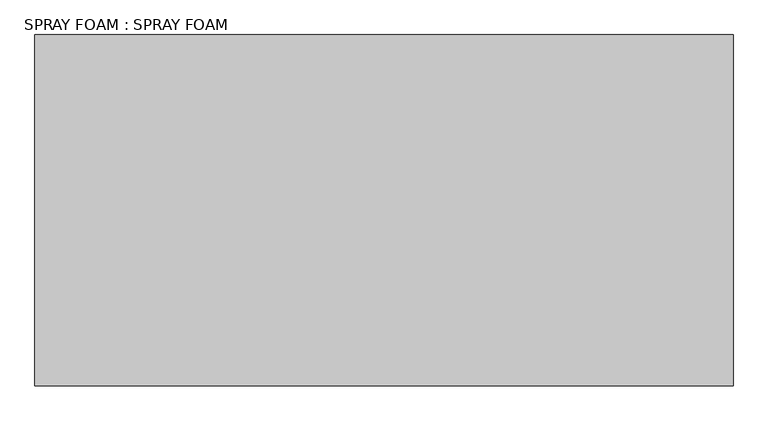
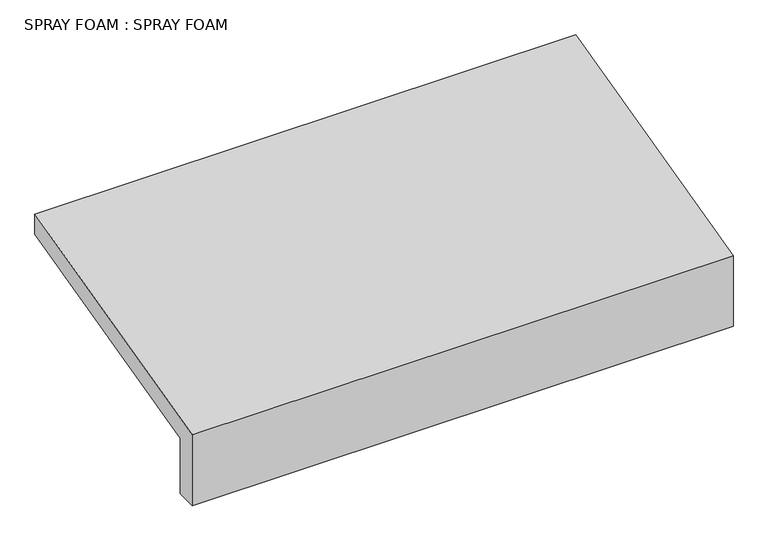
"""IFC4 building model written with IfcOpenShell, lengths in millimetres: proxy geometry, SPRAY FOAM : SPRAY FOAM."""

import ifcopenshell
import ifcopenshell.guid

model = None  # the IFC model being written
_history = None  # IfcOwnerHistory: only IFC2X3 demands one
_inside = {}  # id of a spatial element -> (the spatial element, [elements in it])
_under = {}  # id of a project, library or spatial element -> (it, [spatial elements below it])
_declared = {}  # id of a project -> (the project, [libraries it declares])
_typed = {}  # id of a type object -> (the type object, [elements of that type])
_made_of = {}  # id of a material, layer set ... -> (it, [elements and type objects made of it])


def new_model(schema):
    """Start an empty IFC model of exactly this schema.

    Asked for "IFC4X3", IfcOpenShell would pick the latest addendum, in which some entities
    have other attributes; the version numbers below select the first issue.
    IFC2X3 requires an IfcOwnerHistory on every rooted entity: one is made here for all.
    """
    global model, _history
    if schema == "IFC4X3":
        model = ifcopenshell.file(schema_version=(4, 3, 0, 0))
    else:
        model = ifcopenshell.file(schema=schema)
    _inside.clear()
    _under.clear()
    _declared.clear()
    _typed.clear()
    _made_of.clear()
    _history = None
    if model.schema == "IFC2X3":
        org = make("IfcOrganization", Name="unknown")
        user = make(
            "IfcPersonAndOrganization",
            ThePerson=make("IfcPerson", FamilyName="unknown"),
            TheOrganization=org,
        )
        app = make(
            "IfcApplication",
            ApplicationDeveloper=org,
            Version="unknown",
            ApplicationFullName="unknown",
            ApplicationIdentifier="unknown",
        )
        _history = make(
            "IfcOwnerHistory",
            OwningUser=user,
            OwningApplication=app,
            ChangeAction="ADDED",
            CreationDate=0,
        )
    return model


def make(cls, **values):
    """One entity of the class cls with the attributes given. An attribute that is None is left unset."""
    return model.create_entity(
        cls, **{name: value for name, value in values.items() if value is not None}
    )


def rooted(cls, **values):
    """An entity with a GlobalId (a new one), such as an element, a storey or a relation."""
    return make(cls, GlobalId=ifcopenshell.guid.new(), OwnerHistory=_history, **values)


def si_unit(unit_type, name, prefix=None):
    """IfcSIUnit, for example si_unit("LENGTHUNIT", "METRE", prefix="MILLI")."""
    return make("IfcSIUnit", UnitType=unit_type, Prefix=prefix, Name=name)


def assignment(units):
    """IfcUnitAssignment: the units of a project."""
    return None if units is None else make("IfcUnitAssignment", Units=units)


def point(xyz):
    """IfcCartesianPoint."""
    return None if xyz is None else make("IfcCartesianPoint", Coordinates=xyz)


def direction(xyz):
    """IfcDirection."""
    return None if xyz is None else make("IfcDirection", DirectionRatios=xyz)


def frame(location, z_axis=None, x_axis=None):
    """IfcAxis2Placement3D, a coordinate frame: its origin and axes. An axis left out is left unset."""
    return make(
        "IfcAxis2Placement3D",
        Location=point(location),
        Axis=direction(z_axis),
        RefDirection=direction(x_axis),
    )


def origin():
    """The frame at (0, 0, 0) with its axes left unset."""
    return frame((0.0, 0.0, 0.0))


def place(relative_to, where):
    """IfcLocalPlacement: puts the frame where relative to a parent placement (None: the world)."""
    return make(
        "IfcLocalPlacement", PlacementRelTo=relative_to, RelativePlacement=where
    )


def context(
    kind, dimensions, precision=None, world=None, true_north=None, identifier=None
):
    """IfcGeometricRepresentationContext, for example the 3D "Model" context."""
    return make(
        "IfcGeometricRepresentationContext",
        ContextIdentifier=identifier,
        ContextType=kind,
        CoordinateSpaceDimension=dimensions,
        Precision=precision,
        WorldCoordinateSystem=world,
        TrueNorth=true_north,
    )


def project(units=None, contexts=None):
    """IfcProject with its units and contexts."""
    return rooted(
        "IfcProject",
        Name="project",
        RepresentationContexts=contexts,
        UnitsInContext=assignment(units),
    )


def spatial(cls, under=None, at=None, **own):
    """A site, building, storey or space (cls), placed at a placement, below another one or the project."""
    s = rooted(cls, ObjectPlacement=at, **own)
    if under is not None:
        _under.setdefault(under.id(), (under, []))[1].append(s)
    return s


def polyline(points):
    """IfcPolyline through the points."""
    return make("IfcPolyline", Points=[point(p) for p in points])


def outline(outer, holes=None, kind="AREA"):
    """IfcArbitraryClosedProfileDef: a profile drawn as a closed curve; with holes, ...WithVoids."""
    if holes is None:
        return make("IfcArbitraryClosedProfileDef", ProfileType=kind, OuterCurve=outer)
    return make(
        "IfcArbitraryProfileDefWithVoids",
        ProfileType=kind,
        OuterCurve=outer,
        InnerCurves=holes,
    )


def extrude(swept, where, along, depth):
    """IfcExtrudedAreaSolid: the profile swept, set in the frame where, extruded along a direction by depth."""
    return make(
        "IfcExtrudedAreaSolid",
        SweptArea=swept,
        Position=where,
        ExtrudedDirection=direction(along),
        Depth=depth,
    )


def shape(context_of_items, identifier, shape_type, items):
    """IfcShapeRepresentation: the items that make up one representation, for example the "Body"."""
    return make(
        "IfcShapeRepresentation",
        ContextOfItems=context_of_items,
        RepresentationIdentifier=identifier,
        RepresentationType=shape_type,
        Items=items,
    )


def source(mapping_origin, context_of_items, identifier, shape_type, items):
    """IfcRepresentationMap: a shape defined once, which mapped items show again and again."""
    return make(
        "IfcRepresentationMap",
        MappingOrigin=mapping_origin,
        MappedRepresentation=shape(context_of_items, identifier, shape_type, items),
    )


def transform(
    local_origin,
    x_axis=None,
    y_axis=None,
    z_axis=None,
    scale=None,
    scale2=None,
    scale3=None,
    uniform=True,
):
    """IfcCartesianTransformationOperator3D, or its non-uniform kind. x_axis, y_axis, z_axis: its Axis1, 2, 3."""
    if uniform:
        return make(
            "IfcCartesianTransformationOperator3D",
            Axis1=direction(x_axis),
            Axis2=direction(y_axis),
            LocalOrigin=point(local_origin),
            Scale=scale,
            Axis3=direction(z_axis),
        )
    return make(
        "IfcCartesianTransformationOperator3DnonUniform",
        Axis1=direction(x_axis),
        Axis2=direction(y_axis),
        LocalOrigin=point(local_origin),
        Scale=scale,
        Axis3=direction(z_axis),
        Scale2=scale2,
        Scale3=scale3,
    )


def mapped(mapping_source, mapping_target):
    """IfcMappedItem: shows the shape of a source again, moved by a transform."""
    return make(
        "IfcMappedItem", MappingSource=mapping_source, MappingTarget=mapping_target
    )


def made_of(thing, what):
    """Note that an element or type object is made of a material, layer set ...; save() writes the relation."""
    if what is not None:
        _made_of.setdefault(what.id(), (what, []))[1].append(thing)
    return thing


def element(
    cls,
    number,
    at=None,
    inside=None,
    cuts=None,
    type_object=None,
    material=None,
    context=None,
    identifier="Body",
    shape_type=None,
    held_by="IfcProductDefinitionShape",
    body=None,
    shapes=None,
    **own,
):
    """One element of the class cls, such as IfcWall. Its Tag is "e" and its number.

    at: its placement. inside: the storey or other place that contains it. cuts: it is an
    opening in that element (IfcRelVoidsElement). A single representation is given by context,
    identifier, shape_type and body (its items); several are given by shapes. held_by: the class
    of the entity that holds the representations. save() writes the other relations.
    """
    e = rooted(cls, Tag="e%d" % number, ObjectPlacement=at, **own)
    if body is not None:
        shapes = [shape(context, identifier, shape_type, body)]
    if shapes is not None:
        e.Representation = make(held_by, Representations=shapes)
    if inside is not None:
        _inside.setdefault(inside.id(), (inside, []))[1].append(e)
    if cuts is not None:
        rooted(
            "IfcRelVoidsElement", RelatingBuildingElement=cuts, RelatedOpeningElement=e
        )
    if type_object is not None:
        _typed.setdefault(type_object.id(), (type_object, []))[1].append(e)
    return made_of(e, material)


def aggregate(whole, parts):
    """IfcRelAggregates: a whole, such as a stair, and the parts it consists of."""
    return rooted("IfcRelAggregates", RelatingObject=whole, RelatedObjects=parts)


def save(model, path):
    """Write the relations noted so far, then the file.

    IfcRelAggregates (storeys below a building ...), IfcRelContainedInSpatialStructure (elements
    in a storey), IfcRelDefinesByType, IfcRelAssociatesMaterial and IfcRelDeclares: one each for
    every whole, place, type object, material and project.
    """
    for whole, parts in _under.values():
        aggregate(whole, parts)
    for where, things in _inside.values():
        rooted(
            "IfcRelContainedInSpatialStructure",
            RelatedElements=things,
            RelatingStructure=where,
        )
    for kind, things in _typed.values():
        rooted("IfcRelDefinesByType", RelatedObjects=things, RelatingType=kind)
    for what, things in _made_of.values():
        rooted("IfcRelAssociatesMaterial", RelatedObjects=things, RelatingMaterial=what)
    for by, libraries in _declared.values():
        rooted("IfcRelDeclares", RelatingContext=by, RelatedDefinitions=libraries)
    model.write(path)


def spray_foam_spray_foam_9ee738d7(model_context):
    return source(origin(), model_context, "Body", "SweptSolid", [
        extrude(outline(polyline([(-4275.6279009, 42741.596), (-4351.8279009, 42741.596), (-4351.8279009, 43018.9246048), (-3344.6566162, 43270.717426), (-3344.6566162, 43192.1722638), (-4275.6279009, 42959.4294427), (-4275.6279009, 42741.596)])), frame((12382.7678845, 0.0, 0.0), z_axis=(1.0, 0.0, 0.0), x_axis=(0.0, 1.0, 0.0)), (0.0, 0.0, 1.0), 2000.25),
    ])


if __name__ == "__main__":
    model = new_model("IFC4")
    model_context = context("Model", 3, world=origin())
    ifc_project = project(units=[si_unit("LENGTHUNIT", "METRE", prefix="MILLI")], contexts=[model_context])
    site = spatial("IfcSite", under=ifc_project)
    building = spatial("IfcBuilding", under=site)
    placement = place(None, origin())
    spray_foam_spray_foam_shape = spray_foam_spray_foam_9ee738d7(model_context)
    element("IfcBuildingElementProxy", 1, Name="SPRAY FOAM : SPRAY FOAM", ObjectType="SPRAY FOAM : SPRAY FOAM", at=placement, inside=building, context=model_context, shape_type="MappedRepresentation", body=[
        mapped(spray_foam_spray_foam_shape, transform((0.0, 0.0, 0.0), x_axis=(1.0, 0.0, 0.0), y_axis=(0.0, 1.0, 0.0), z_axis=(0.0, 0.0, 1.0))),
    ])
    save(model, "model.ifc")

# Revit data of these elements
# Type "SPRAY FOAM : SPRAY FOAM"
#   NameOverride = "SPRAY FOAM"
# Element 1 (IfcBuildingElementProxy, "SPRAY FOAM : SPRAY FOAM")
#   Materials on its faces: "POLYURETHANE SPRAY FOAM UNDER ROOF SUBSTRATE (SEE T-24 ENERGY REPORT FOR R-VALUE)"
# Materials
#   "POLYURETHANE SPRAY FOAM UNDER ROOF SUBSTRATE (SEE T-24 ENERGY REPORT FOR R-VALUE)": class "Unassigned", colour RGB 210 164 194, transparency 0, Cost = 0
